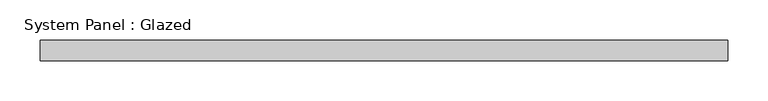
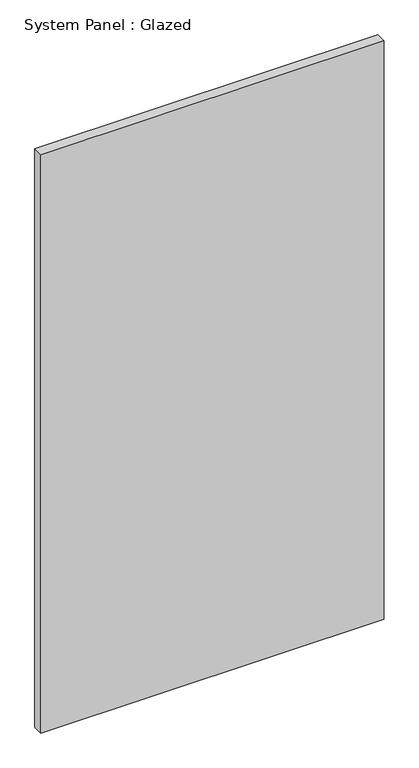
"""IFC4 building model written with IfcOpenShell, lengths in millimetres: plate geometry, System Panel : Glazed."""

from ifc_helpers import new_model, si_unit, origin, origin_with_axes, place, context, project, spatial, polyline, outline, extrude, source, transform, mapped, element, save


def system_panel_glazed_ccfd9adb(model_context):
    return source(origin(), model_context, "Body", "SweptSolid", [
        extrude(outline(polyline([(427.9999998, 19.05), (-427.9999998, 19.05), (-427.9999998, 44.45), (427.9999998, 44.45), (427.9999998, 19.05)])), origin_with_axes(), (0.0, 0.0, 1.0), 1524.0),
    ])


if __name__ == "__main__":
    model = new_model("IFC4")
    model_context = context("Model", 3, world=origin())
    ifc_project = project(units=[si_unit("LENGTHUNIT", "METRE", prefix="MILLI")], contexts=[model_context])
    site = spatial("IfcSite", under=ifc_project)
    building = spatial("IfcBuilding", under=site)
    placement = place(None, origin())
    system_panel_glazed_shape = system_panel_glazed_ccfd9adb(model_context)
    element("IfcPlate", 1, ObjectType="System Panel : Glazed", at=placement, inside=building, context=model_context, shape_type="MappedRepresentation", body=[
        mapped(system_panel_glazed_shape, transform((0.0, 0.0, 0.0), x_axis=(1.0, 0.0, 0.0), y_axis=(0.0, 1.0, 0.0), z_axis=(0.0, 0.0, 1.0))),
    ])
    save(model, "model.ifc")

# Revit data of these elements
# Type "System Panel : Glazed"
#   Construction Type Id = "GSP4R"
#   Analytic Construction = "1/8 in Pilkington single glazing"
#   Visual Light Transmittance = 0.9
#   Solar Heat Gain Coefficient = 0.86
#   Heat Transfer Coefficient (U) = 6.7069 W/(m²·K)
# Element 1 (IfcPlate, "System Panel : Glazed")
#   Materials on its faces: "Glass"
# Materials
#   "Glass": class "Glass", colour RGB 0 128 192, transparency 0.75, Description = "Soda Lime Glass", Cost = 0
